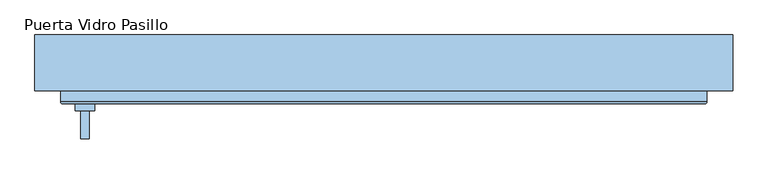
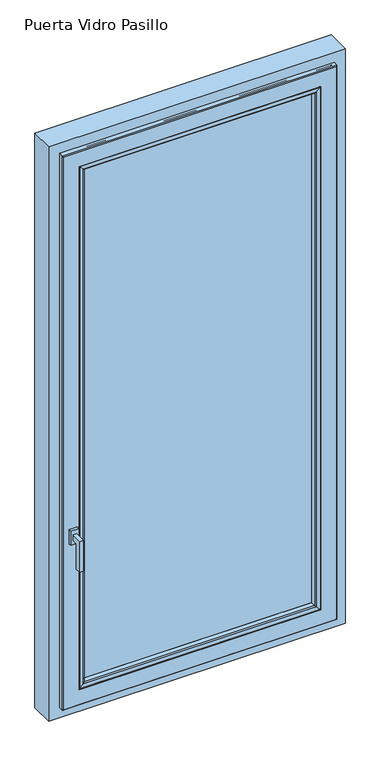
"""IFC4 building model written with IfcOpenShell, lengths in millimetres: window geometry, 2019_ES_Ventana_Replus_re80pvc301_10100_1-Hoja : Puerta Vidro Pasillo."""

from ifc_helpers import new_model, si_unit, frame, origin, place, context, project, spatial, polyline, ellipse_curve, outline, extrude, source, transform, mapped, element, save
from ifc_brep_helpers import plane_surface, cylinder_surface, advanced_brep


def puerta_vidro_pasillo_571ac3f6(model_context):
    return source(origin(), model_context, "Body", "SolidModel", [
        extrude(outline(polyline([(-78.4999991, 1470.0), (-78.4999991, 1450.0), (-98.4999991, 1450.0), (-98.4999991, 1360.0), (-118.4999991, 1360.0), (-118.4999991, 1470.0), (-78.4999991, 1470.0)])), frame((-434.1999993, 0.0, 0.0), z_axis=(1.0, 0.0, 0.0), x_axis=(0.0, 1.0, 0.0)), (0.0, 0.0, 1.0), 12.0),
        extrude(outline(polyline([(-413.9687607, -78.4999991), (-442.4312378, -78.4999991), (-442.4312378, -68.4999991), (-413.9687607, -68.4999991), (-413.9687607, -78.4999991)])), frame((0.0, 0.0, 1435.217127), z_axis=(0.0, 0.0, 1.0), x_axis=(1.0, 0.0, 0.0)), (0.0, 0.0, 1.0), 49.565746),
        extrude(outline(polyline([(2757.2, 397.1999993), (2757.2, -397.1999993), (909.8, -397.1999993), (909.8, 397.1999993), (2757.2, 397.1999993)]), holes=[polyline([(917.8, 389.1999993), (917.8, -389.1999993), (2749.2, -389.1999993), (2749.2, 389.1999993), (917.8, 389.1999993)])]), frame((0.0, -26.9999999, 0.0), z_axis=(0.0, 1.0, 0.0), x_axis=(0.0, 0.0, 1.0)), (0.0, 0.0, 1.0), 16.0),
        extrude(outline(polyline([(2757.1868066, 397.1868058), (2757.1868066, -397.1868058), (909.8131934, -397.1868058), (909.8131934, 397.1868058), (2757.1868066, 397.1868058)]), holes=[polyline([(917.8, 389.1999993), (917.8, -389.1999993), (2749.2, -389.1999993), (2749.2, 389.1999993), (917.8, 389.1999993)])]), frame((0.0, -47.0000001, 0.0), z_axis=(0.0, 1.0, 0.0), x_axis=(0.0, 0.0, 1.0)), (0.0, 0.0, 1.0), 16.0),
        extrude(outline(polyline([(397.1999993, -6.9999997), (397.1999993, -10.9999999), (-397.1999993, -10.9999999), (-397.1999993, -6.9999997), (397.1999993, -6.9999997)])), frame((0.0, 0.0, 903.7946451), z_axis=(0.0, 0.0, 1.0), x_axis=(1.0, 0.0, 0.0)), (0.0, 0.0, 1.0), 1859.4053549),
        extrude(outline(polyline([(397.1999993, -26.9999999), (397.1999993, -31.0000001), (-397.1999993, -31.0000001), (-397.1999993, -26.9999999), (397.1999993, -26.9999999)])), frame((0.0, 0.0, 903.7946451), z_axis=(0.0, 0.0, 1.0), x_axis=(1.0, 0.0, 0.0)), (0.0, 0.0, 1.0), 1859.4053549),
        extrude(outline(polyline([(397.1999993, -47.0000001), (397.1999993, -51.0000003), (-397.1999993, -51.0000003), (-397.1999993, -47.0000001), (397.1999993, -47.0000001)])), frame((0.0, 0.0, 903.7946451), z_axis=(0.0, 0.0, 1.0), x_axis=(1.0, 0.0, 0.0)), (0.0, 0.0, 1.0), 1859.4053549),
        advanced_brep(
        [(387.2913171, 9.2764571, 2747.2913178), (390.1890946, 11.5, 2750.1890953), (390.1890946, 11.5, 919.8109047), (387.2913171, 9.2764571, 922.7086822), (430.1999993, 11.5, 879.8), (-430.1999993, 11.5, 879.8), (-430.1999993, 11.5, 2790.2), (430.1999993, 11.5, 2790.2), (-390.1890946, 11.5, 2750.1890953), (-390.1890946, 11.5, 919.8109047), (-387.2913171, 9.2764571, 922.7086822), (384.1757968, -2.3508228, 2744.1757976), (384.1757968, -2.3508228, 925.8242024), (-384.1757968, -2.3508228, 925.8242024), (384.6739305, -3.0000033, 2744.6739313), (384.6739305, -3.0000033, 925.3260687), (-384.6739305, -3.0000033, 925.3260687), (391.1999993, -3.0000033, 2751.2), (-391.1999993, -3.0000033, 2751.2), (-391.1999993, -3.0000033, 918.8), (391.1999993, -3.0000033, 918.8), (-384.6739305, -3.0000033, 2744.6739313), (391.1999993, -6.9999997, 2751.2), (391.1999993, -6.9999997, 918.8), (-391.1999993, -6.9999997, 918.8), (411.8162192, -6.9999997, 2771.8162199), (-411.8162192, -6.9999997, 2771.8162199), (-411.8162192, -6.9999997, 898.1837801), (411.8162192, -6.9999997, 898.1837801), (-391.1999993, -6.9999997, 2751.2), (409.1999993, -25.6153717, 2769.2), (409.1999993, -25.6153717, 900.8), (-409.1999993, -25.6153717, 900.8), (409.1999993, -56.4999995, 2769.2), (409.1999993, -56.4999995, 900.8), (-409.1999993, -56.4999995, 900.8), (-409.1999993, -56.4999995, 2769.2), (397.1999993, -56.4999995, 2757.2), (-397.1999993, -56.4999995, 2757.2), (-397.1999993, -56.4999995, 912.8), (397.1999993, -56.4999995, 912.8), (397.1999993, -51.0000003, 2757.2), (397.1999993, -51.0000003, 912.8), (-397.1999993, -51.0000003, 912.8), (-397.1999993, -51.0000003, 2757.2), (386.007687, -51.0000003, 2746.0076877), (-386.007687, -51.0000003, 2746.0076877), (-386.007687, -51.0000003, 923.9923123), (386.007687, -51.0000003, 923.9923123), (385.4940999, -51.6693201, 2745.4941006), (385.4940999, -51.6693201, 924.5058994), (-385.4940999, -51.6693201, 924.5058994), (388.8993918, -64.3780426, 2748.8993925), (388.8993918, -64.3780426, 921.1006075), (-388.8993918, -64.3780426, 921.1006075), (392.6234971, -67.3403297, 2752.6234978), (392.6234971, -67.3403297, 917.3765022), (-392.6234971, -67.3403297, 917.3765022), (405.6488427, -67.7951848, 2765.6488434), (405.6488427, -67.7951848, 904.3511566), (-405.6488427, -67.7951848, 904.3511566), (406.1999993, -67.2629391, 2766.2), (406.1999993, -67.2629391, 903.8), (-406.1999993, -67.2629391, 903.8), (407.4370593, -68.4999991, 2767.43706), (407.4370593, -68.4999991, 902.56294), (-407.4370593, -68.4999991, 902.56294), (460.1999993, -68.4999991, 2820.2), (-460.1999993, -68.4999991, 2820.2), (-460.1999993, -68.4999991, 849.8), (460.1999993, -68.4999991, 849.8), (-407.4370593, -68.4999991, 2767.43706), (463.1999993, -65.4999991, 2823.2), (463.1999993, -65.4999991, 846.8), (-463.1999993, -65.4999991, 846.8), (463.1999993, -50.0, 2823.2), (463.1999993, -50.0, 846.8), (-463.1999993, -50.0, 846.8), (-463.1999993, -50.0, 2823.2), (443.1999993, -50.0, 2803.2), (-443.1999993, -50.0, 2803.2), (-443.1999993, -50.0, 866.8), (443.1999993, -50.0, 866.8), (443.1999993, -11.9999991, 866.8), (443.1999993, -11.9999991, 2803.2), (-443.1999993, -11.9999991, 866.8), (-443.1999993, -11.9999991, 2803.2), (430.1999993, -11.9999991, 2790.2), (-430.1999993, -11.9999991, 2790.2), (-430.1999993, -11.9999991, 879.8), (430.1999993, -11.9999991, 879.8), (-387.2913171, 9.2764571, 2747.2913178), (-384.1757968, -2.3508228, 2744.1757976), (-409.1999993, -25.6153717, 2769.2), (-385.4940999, -51.6693201, 2745.4941006), (-388.8993918, -64.3780426, 2748.8993925), (-392.6234971, -67.3403297, 2752.6234978), (-405.6488427, -67.7951848, 2765.6488434), (-406.1999993, -67.2629391, 2766.2), (-463.1999993, -65.4999991, 2823.2)],
        [
            (0, 1, ellipse_curve(frame((390.1890946, 8.5, 2750.1890953), z_axis=(0.7071067811865475, 0.0, -0.7071067811865475), x_axis=(0.7071067811865474, 0.0, 0.7071067811865476)), 4.2426407, 3.0)),
            (1, 2),
            (2, 3, ellipse_curve(frame((390.1890946, 8.5, 919.8109047), z_axis=(0.7071067811865475, 0.0, 0.7071067811865475), x_axis=(-0.7071067811865474, 0.0, 0.7071067811865476)), 4.2426407, 3.0)),
            (3, 0),
            (4, 5),
            (5, 6),
            (6, 7),
            (7, 4),
            (1, 8),
            (8, 9),
            (9, 2),
            (9, 10, ellipse_curve(frame((-390.1890946, 8.5, 919.8109047), z_axis=(0.7071067811865475, 0.0, -0.7071067811865475), x_axis=(0.7071067811865476, 0.0, 0.7071067811865474)), 4.2426407, 3.0)),
            (10, 3),
            (11, 0),
            (3, 12),
            (12, 11),
            (10, 13),
            (13, 12),
            (14, 11, ellipse_curve(frame((384.6739305, -2.4842973, 2744.6739313), z_axis=(0.7071067811865475, 0.0, -0.7071067811865475), x_axis=(0.7071067811865474, 0.0, 0.7071067811865476)), 0.7293184, 0.515706)),
            (12, 15, ellipse_curve(frame((384.6739305, -2.4842973, 925.3260687), z_axis=(0.7071067811865475, 0.0, 0.7071067811865475), x_axis=(-0.7071067811865474, 0.0, 0.7071067811865476)), 0.7293184, 0.515706)),
            (15, 14),
            (13, 16, ellipse_curve(frame((-384.6739305, -2.4842973, 925.3260687), z_axis=(0.7071067811865475, 0.0, -0.7071067811865475), x_axis=(0.7071067811865476, 0.0, 0.7071067811865474)), 0.7293184, 0.515706)),
            (16, 15),
            (17, 18),
            (18, 19),
            (19, 20),
            (20, 17),
            (16, 21),
            (21, 14),
            (22, 17),
            (20, 23),
            (23, 22),
            (19, 24),
            (24, 23),
            (25, 26),
            (26, 27),
            (27, 28),
            (28, 25),
            (24, 29),
            (29, 22),
            (30, 25),
            (28, 31),
            (31, 30),
            (27, 32),
            (32, 31),
            (33, 30),
            (31, 34),
            (34, 33),
            (32, 35),
            (35, 34),
            (35, 36),
            (36, 33),
            (37, 38),
            (38, 39),
            (39, 40),
            (40, 37),
            (41, 37),
            (40, 42),
            (42, 41),
            (39, 43),
            (43, 42),
            (43, 44),
            (44, 41),
            (45, 46),
            (46, 47),
            (47, 48),
            (48, 45),
            (49, 45, ellipse_curve(frame((386.007687, -51.5317048, 2746.0076877), z_axis=(0.7071067811865475, 0.0, -0.7071067811865475), x_axis=(0.7071067811865474, 0.0, 0.7071067811865476)), 0.7519437, 0.5317045)),
            (48, 50, ellipse_curve(frame((386.007687, -51.5317048, 923.9923123), z_axis=(0.7071067811865475, 0.0, 0.7071067811865475), x_axis=(-0.7071067811865474, 0.0, 0.7071067811865476)), 0.7519437, 0.5317045)),
            (50, 49),
            (47, 51, ellipse_curve(frame((-386.007687, -51.5317048, 923.9923123), z_axis=(0.7071067811865475, 0.0, -0.7071067811865475), x_axis=(0.7071067811865476, 0.0, 0.7071067811865474)), 0.7519437, 0.5317045)),
            (51, 50),
            (52, 49),
            (50, 53),
            (53, 52),
            (51, 54),
            (54, 53),
            (55, 52, ellipse_curve(frame((392.7630951, -63.3427664, 2752.7630958), z_axis=(0.7071067811865475, 0.0, -0.7071067811865475), x_axis=(0.7071067811865474, 0.0, 0.7071067811865476)), 5.6568542, 4.0)),
            (53, 56, ellipse_curve(frame((392.7630951, -63.3427664, 917.2369042), z_axis=(0.7071067811865475, 0.0, 0.7071067811865475), x_axis=(-0.7071067811865474, 0.0, 0.7071067811865476)), 5.6568542, 4.0)),
            (56, 55),
            (54, 57, ellipse_curve(frame((-392.7630951, -63.3427664, 917.2369042), z_axis=(0.7071067811865475, 0.0, -0.7071067811865475), x_axis=(0.7071067811865476, 0.0, 0.7071067811865474)), 5.6568542, 4.0)),
            (57, 56),
            (58, 55),
            (56, 59),
            (59, 58),
            (57, 60),
            (60, 59),
            (61, 58, ellipse_curve(frame((405.6674291, -67.2629391, 2765.6674299), z_axis=(0.7071067811865475, 0.0, -0.7071067811865475), x_axis=(0.7071067811865474, 0.0, 0.7071067811865476)), 0.7531679, 0.5325701)),
            (59, 62, ellipse_curve(frame((405.6674291, -67.2629391, 904.3325701), z_axis=(0.7071067811865475, 0.0, 0.7071067811865475), x_axis=(-0.7071067811865474, 0.0, 0.7071067811865476)), 0.7531679, 0.5325701)),
            (62, 61),
            (60, 63, ellipse_curve(frame((-405.6674291, -67.2629391, 904.3325701), z_axis=(0.7071067811865475, 0.0, -0.7071067811865475), x_axis=(0.7071067811865476, 0.0, 0.7071067811865474)), 0.7531679, 0.5325701)),
            (63, 62),
            (64, 61, ellipse_curve(frame((407.4370593, -67.2629391, 2767.43706), z_axis=(0.7071067811865475, 0.0, -0.7071067811865475), x_axis=(0.7071067811865474, 0.0, 0.7071067811865476)), 1.7494671, 1.23706)),
            (62, 65, ellipse_curve(frame((407.4370593, -67.2629391, 902.56294), z_axis=(0.7071067811865475, 0.0, 0.7071067811865475), x_axis=(-0.7071067811865474, 0.0, 0.7071067811865476)), 1.7494671, 1.23706)),
            (65, 64),
            (63, 66, ellipse_curve(frame((-407.4370593, -67.2629391, 902.56294), z_axis=(0.7071067811865475, 0.0, -0.7071067811865475), x_axis=(0.7071067811865476, 0.0, 0.7071067811865474)), 1.7494671, 1.23706)),
            (66, 65),
            (67, 68),
            (68, 69),
            (69, 70),
            (70, 67),
            (66, 71),
            (71, 64),
            (72, 67, ellipse_curve(frame((460.1999993, -65.4999991, 2820.2), z_axis=(0.7071067811865475, 0.0, -0.7071067811865475), x_axis=(0.7071067811865474, 0.0, 0.7071067811865476)), 4.2426407, 3.0)),
            (70, 73, ellipse_curve(frame((460.1999993, -65.4999991, 849.8), z_axis=(0.7071067811865475, 0.0, 0.7071067811865475), x_axis=(-0.7071067811865474, 0.0, 0.7071067811865476)), 4.2426407, 3.0)),
            (73, 72),
            (69, 74, ellipse_curve(frame((-460.1999993, -65.4999991, 849.8), z_axis=(0.7071067811865475, 0.0, -0.7071067811865475), x_axis=(0.7071067811865476, 0.0, 0.7071067811865474)), 4.2426407, 3.0)),
            (74, 73),
            (75, 72),
            (73, 76),
            (76, 75),
            (74, 77),
            (77, 76),
            (77, 78),
            (78, 75),
            (79, 80),
            (80, 81),
            (81, 82),
            (82, 79),
            (82, 83),
            (83, 84),
            (84, 79),
            (81, 85),
            (85, 83),
            (85, 86),
            (86, 84),
            (87, 88),
            (88, 89),
            (89, 90),
            (90, 87),
            (90, 4),
            (7, 87),
            (89, 5),
            (8, 91, ellipse_curve(frame((-390.1890946, 8.5, 2750.1890953), z_axis=(-0.7071067811865475, 0.0, -0.7071067811865475), x_axis=(0.7071067811865474, 0.0, -0.7071067811865476)), 4.2426407, 3.0)),
            (91, 10),
            (91, 92),
            (92, 13),
            (92, 21, ellipse_curve(frame((-384.6739305, -2.4842973, 2744.6739313), z_axis=(-0.7071067811865475, 0.0, -0.7071067811865475), x_axis=(0.7071067811865474, 0.0, -0.7071067811865476)), 0.7293184, 0.515706)),
            (18, 29),
            (26, 93),
            (93, 32),
            (93, 36),
            (38, 44),
            (46, 94, ellipse_curve(frame((-386.007687, -51.5317048, 2746.0076877), z_axis=(-0.7071067811865475, 0.0, -0.7071067811865475), x_axis=(0.7071067811865474, 0.0, -0.7071067811865476)), 0.7519437, 0.5317045)),
            (94, 51),
            (94, 95),
            (95, 54),
            (95, 96, ellipse_curve(frame((-392.7630951, -63.3427664, 2752.7630958), z_axis=(-0.7071067811865475, 0.0, -0.7071067811865475), x_axis=(0.7071067811865474, 0.0, -0.7071067811865476)), 5.6568542, 4.0)),
            (96, 57),
            (96, 97),
            (97, 60),
            (97, 98, ellipse_curve(frame((-405.6674291, -67.2629391, 2765.6674299), z_axis=(-0.7071067811865475, 0.0, -0.7071067811865475), x_axis=(0.7071067811865474, 0.0, -0.7071067811865476)), 0.7531679, 0.5325701)),
            (98, 63),
            (98, 71, ellipse_curve(frame((-407.4370593, -67.2629391, 2767.43706), z_axis=(-0.7071067811865475, 0.0, -0.7071067811865475), x_axis=(0.7071067811865474, 0.0, -0.7071067811865476)), 1.7494671, 1.23706)),
            (68, 99, ellipse_curve(frame((-460.1999993, -65.4999991, 2820.2), z_axis=(-0.7071067811865475, 0.0, -0.7071067811865475), x_axis=(0.7071067811865474, 0.0, -0.7071067811865476)), 4.2426407, 3.0)),
            (99, 74),
            (99, 78),
            (80, 86),
            (88, 6),
            (0, 91),
            (11, 92),
            (30, 93),
            (49, 94),
            (52, 95),
            (55, 96),
            (58, 97),
            (61, 98),
            (72, 99),
        ],
        [
            cylinder_surface(frame((390.1890946, 8.5, 2823.2), z_axis=(0.0, 0.0, 1.0), x_axis=(-1.0, 0.0, 0.0)), 3.0),
            plane_surface(frame((-430.1999993, 11.5, 2790.2), z_axis=(0.0, 1.0, 0.0), x_axis=(1.0, 0.0, 0.0))),
            cylinder_surface(frame((463.1999993, 8.5, 919.8109047), z_axis=(1.0, 0.0, 0.0), x_axis=(0.0, 0.0, 1.0)), 3.0),
            plane_surface(frame((387.2913171, 9.2764571, 2747.2913178), z_axis=(-0.9659258263570549, 0.2588190448487916, 0.0), x_axis=(0.0, 0.0, -1.0))),
            plane_surface(frame((387.2913171, 9.2764571, 922.7086822), z_axis=(0.0, 0.2588190448487885, 0.9659258263570558), x_axis=(-1.0, 0.0, 0.0))),
            cylinder_surface(frame((384.6739305, -2.4842973, 2823.2), z_axis=(0.0, 0.0, 1.0), x_axis=(-1.0, 0.0, 0.0)), 0.515706),
            cylinder_surface(frame((463.1999993, -2.4842973, 925.3260687), z_axis=(1.0, 0.0, 0.0), x_axis=(0.0, 0.0, 1.0)), 0.515706),
            plane_surface(frame((-384.6739305, -3.0000033, 2744.6739313), z_axis=(0.0, -1.0, 0.0), x_axis=(1.0, 0.0, 0.0))),
            plane_surface(frame((391.1999993, -3.0000033, 2751.2), z_axis=(-1.0, 0.0, 0.0), x_axis=(0.0, 0.0, -1.0))),
            plane_surface(frame((391.1999993, -3.0000033, 918.8), z_axis=(0.0, 0.0, 1.0), x_axis=(-1.0, 0.0, 0.0))),
            plane_surface(frame((-391.1999993, -6.9999997, 2751.2), z_axis=(0.0, -1.0, 0.0), x_axis=(1.0, 0.0, 0.0))),
            plane_surface(frame((411.8162192, -6.9999997, 2771.8162199), z_axis=(-0.9902680687415736, 0.13917310096004265, 0.0), x_axis=(0.0, 0.0, -1.0))),
            plane_surface(frame((411.8162192, -6.9999997, 898.1837801), z_axis=(0.0, 0.13917310096003946, 0.990268068741574), x_axis=(-1.0, 0.0, 0.0))),
            plane_surface(frame((409.1999993, -25.6153717, 2769.2), z_axis=(-1.0, 0.0, 0.0), x_axis=(0.0, 0.0, -1.0))),
            plane_surface(frame((409.1999993, -25.6153717, 900.8), z_axis=(0.0, 0.0, 1.0), x_axis=(-1.0, 0.0, 0.0))),
            plane_surface(frame((-409.1999993, -56.4999995, 2769.2), z_axis=(0.0, 1.0, 0.0), x_axis=(1.0, 0.0, 0.0))),
            plane_surface(frame((397.1999993, -56.4999995, 2757.2), z_axis=(1.0, 0.0, 0.0), x_axis=(0.0, 0.0, -1.0))),
            plane_surface(frame((397.1999993, -56.4999995, 912.8), z_axis=(0.0, 0.0, -1.0), x_axis=(-1.0, 0.0, 0.0))),
            plane_surface(frame((-397.1999993, -51.0000003, 2757.2), z_axis=(0.0, 1.0, 0.0), x_axis=(1.0, 0.0, 0.0))),
            cylinder_surface(frame((386.007687, -51.5317048, 2823.2), z_axis=(0.0, 0.0, 1.0), x_axis=(-1.0, 0.0, 0.0)), 0.5317045),
            cylinder_surface(frame((463.1999993, -51.5317048, 923.9923123), z_axis=(1.0, 0.0, 0.0), x_axis=(0.0, 0.0, 1.0)), 0.5317045),
            plane_surface(frame((385.4940999, -51.6693201, 2745.4941006), z_axis=(-0.9659258262890666, -0.2588190451025272, 0.0), x_axis=(0.0, 0.0, -1.0))),
            plane_surface(frame((385.4940999, -51.6693201, 924.5058994), z_axis=(0.0, -0.2588190451025303, 0.9659258262890658), x_axis=(-1.0, 0.0, 0.0))),
            cylinder_surface(frame((392.7630951, -63.3427664, 2823.2), z_axis=(0.0, 0.0, 1.0), x_axis=(-1.0, 0.0, 0.0)), 4.0),
            cylinder_surface(frame((463.1999993, -63.3427664, 917.2369042), z_axis=(1.0, 0.0, 0.0), x_axis=(0.0, 0.0, 1.0)), 4.0),
            plane_surface(frame((392.6234971, -67.3403297, 2752.6234978), z_axis=(-0.034899496702507804, -0.9993908270190955, 0.0), x_axis=(0.0, 0.0, -1.0))),
            plane_surface(frame((392.6234971, -67.3403297, 917.3765022), z_axis=(0.0, -0.9993908270190957, 0.03489949670250457), x_axis=(-1.0, 0.0, 0.0))),
            cylinder_surface(frame((405.6674291, -67.2629391, 2823.2), z_axis=(0.0, 0.0, 1.0), x_axis=(-1.0, 0.0, 0.0)), 0.5325701),
            cylinder_surface(frame((463.1999993, -67.2629391, 904.3325701), z_axis=(1.0, 0.0, 0.0), x_axis=(0.0, 0.0, 1.0)), 0.5325701),
            cylinder_surface(frame((407.4370593, -67.2629391, 2823.2), z_axis=(0.0, 0.0, 1.0), x_axis=(-1.0, 0.0, 0.0)), 1.23706),
            cylinder_surface(frame((463.1999993, -67.2629391, 902.56294), z_axis=(1.0, 0.0, 0.0), x_axis=(0.0, 0.0, 1.0)), 1.23706),
            plane_surface(frame((-407.4370593, -68.4999991, 2767.43706), z_axis=(0.0, -1.0, 0.0), x_axis=(1.0, 0.0, 0.0))),
            cylinder_surface(frame((460.1999993, -65.4999991, 2823.2), z_axis=(0.0, 0.0, 1.0), x_axis=(-1.0, 0.0, 0.0)), 3.0),
            cylinder_surface(frame((463.1999993, -65.4999991, 849.8), z_axis=(1.0, 0.0, 0.0), x_axis=(0.0, 0.0, 1.0)), 3.0),
            plane_surface(frame((463.1999993, -65.4999991, 2823.2), z_axis=(1.0, 0.0, 0.0), x_axis=(0.0, 0.0, -1.0))),
            plane_surface(frame((463.1999993, -65.4999991, 846.8), z_axis=(0.0, 0.0, -1.0), x_axis=(-1.0, 0.0, 0.0))),
            plane_surface(frame((-459.2000019, -50.0, 2819.2000027), z_axis=(0.0, 1.0, 0.0), x_axis=(1.0, 0.0, 0.0))),
            plane_surface(frame((443.1999993, -45.0999991, 2803.2), z_axis=(1.0, 0.0, 0.0), x_axis=(0.0, 0.0, -1.0))),
            plane_surface(frame((443.1999993, -45.0999991, 866.8), z_axis=(0.0, 0.0, -1.0), x_axis=(-1.0, 0.0, 0.0))),
            plane_surface(frame((-435.7000002, -11.9999991, 2795.7000009), z_axis=(0.0, 1.0, 0.0), x_axis=(1.0, 0.0, 0.0))),
            plane_surface(frame((430.1999993, -1.4999991, 2790.2), z_axis=(1.0, 0.0, 0.0), x_axis=(0.0, 0.0, -1.0))),
            plane_surface(frame((430.1999993, -1.4999991, 879.8), z_axis=(0.0, 0.0, -1.0), x_axis=(-1.0, 0.0, 0.0))),
            cylinder_surface(frame((-390.1890946, 8.5, 846.8), z_axis=(0.0, 0.0, -1.0), x_axis=(1.0, 0.0, 0.0)), 3.0),
            plane_surface(frame((-387.2913171, 9.2764571, 922.7086822), z_axis=(0.9659258263570565, 0.2588190448487853, 0.0), x_axis=(0.0, 0.0, 1.0))),
            cylinder_surface(frame((-384.6739305, -2.4842973, 846.8), z_axis=(0.0, 0.0, -1.0), x_axis=(1.0, 0.0, 0.0)), 0.515706),
            plane_surface(frame((-391.1999993, -3.0000033, 918.8), z_axis=(1.0, 0.0, 0.0), x_axis=(0.0, 0.0, 1.0))),
            plane_surface(frame((-411.8162192, -6.9999997, 898.1837801), z_axis=(0.9902680687415745, 0.13917310096003627, 0.0), x_axis=(0.0, 0.0, 1.0))),
            plane_surface(frame((-409.1999993, -25.6153717, 900.8), z_axis=(1.0, 0.0, 0.0), x_axis=(0.0, 0.0, 1.0))),
            plane_surface(frame((-397.1999993, -56.4999995, 912.8), z_axis=(-1.0, 0.0, 0.0), x_axis=(0.0, 0.0, 1.0))),
            cylinder_surface(frame((-386.007687, -51.5317048, 846.8), z_axis=(0.0, 0.0, -1.0), x_axis=(1.0, 0.0, 0.0)), 0.5317045),
            plane_surface(frame((-385.4940999, -51.6693201, 924.5058994), z_axis=(0.9659258262890649, -0.2588190451025334, 0.0), x_axis=(0.0, 0.0, 1.0))),
            cylinder_surface(frame((-392.7630951, -63.3427664, 846.8), z_axis=(0.0, 0.0, -1.0), x_axis=(1.0, 0.0, 0.0)), 4.0),
            plane_surface(frame((-392.6234971, -67.3403297, 917.3765022), z_axis=(0.03489949670250134, -0.9993908270190958, 0.0), x_axis=(0.0, 0.0, 1.0))),
            cylinder_surface(frame((-405.6674291, -67.2629391, 846.8), z_axis=(0.0, 0.0, -1.0), x_axis=(1.0, 0.0, 0.0)), 0.5325701),
            cylinder_surface(frame((-407.4370593, -67.2629391, 846.8), z_axis=(0.0, 0.0, -1.0), x_axis=(1.0, 0.0, 0.0)), 1.23706),
            cylinder_surface(frame((-460.1999993, -65.4999991, 846.8), z_axis=(0.0, 0.0, -1.0), x_axis=(1.0, 0.0, 0.0)), 3.0),
            plane_surface(frame((-463.1999993, -65.4999991, 846.8), z_axis=(-1.0, 0.0, 0.0), x_axis=(0.0, 0.0, 1.0))),
            plane_surface(frame((-443.1999993, -45.0999991, 866.8), z_axis=(-1.0, 0.0, 0.0), x_axis=(0.0, 0.0, 1.0))),
            plane_surface(frame((-430.1999993, -1.4999991, 879.8), z_axis=(-1.0, 0.0, 0.0), x_axis=(0.0, 0.0, 1.0))),
            cylinder_surface(frame((-463.1999993, 8.5, 2750.1890953), z_axis=(-1.0, 0.0, 0.0), x_axis=(0.0, 0.0, -1.0)), 3.0),
            plane_surface(frame((-387.2913171, 9.2764571, 2747.2913178), z_axis=(0.0, 0.2588190448487885, -0.9659258263570557), x_axis=(1.0, 0.0, 0.0))),
            cylinder_surface(frame((-463.1999993, -2.4842973, 2744.6739313), z_axis=(-1.0, 0.0, 0.0), x_axis=(0.0, 0.0, -1.0)), 0.515706),
            plane_surface(frame((-391.1999993, -3.0000033, 2751.2), z_axis=(0.0, 0.0, -1.0), x_axis=(1.0, 0.0, 0.0))),
            plane_surface(frame((-411.8162192, -6.9999997, 2771.8162199), z_axis=(0.0, 0.13917310096003946, -0.990268068741574), x_axis=(1.0, 0.0, 0.0))),
            plane_surface(frame((-409.1999993, -25.6153717, 2769.2), z_axis=(0.0, 0.0, -1.0), x_axis=(1.0, 0.0, 0.0))),
            plane_surface(frame((-397.1999993, -56.4999995, 2757.2), z_axis=(0.0, 0.0, 1.0), x_axis=(1.0, 0.0, 0.0))),
            cylinder_surface(frame((-463.1999993, -51.5317048, 2746.0076877), z_axis=(-1.0, 0.0, 0.0), x_axis=(0.0, 0.0, -1.0)), 0.5317045),
            plane_surface(frame((-385.4940999, -51.6693201, 2745.4941006), z_axis=(0.0, -0.2588190451025303, -0.9659258262890658), x_axis=(1.0, 0.0, 0.0))),
            cylinder_surface(frame((-463.1999993, -63.3427664, 2752.7630958), z_axis=(-1.0, 0.0, 0.0), x_axis=(0.0, 0.0, -1.0)), 4.0),
            plane_surface(frame((-392.6234971, -67.3403297, 2752.6234978), z_axis=(0.0, -0.9993908270190957, -0.03489949670250457), x_axis=(1.0, 0.0, 0.0))),
            cylinder_surface(frame((-463.1999993, -67.2629391, 2765.6674299), z_axis=(-1.0, 0.0, 0.0), x_axis=(0.0, 0.0, -1.0)), 0.5325701),
            cylinder_surface(frame((-463.1999993, -67.2629391, 2767.43706), z_axis=(-1.0, 0.0, 0.0), x_axis=(0.0, 0.0, -1.0)), 1.23706),
            cylinder_surface(frame((-463.1999993, -65.4999991, 2820.2), z_axis=(-1.0, 0.0, 0.0), x_axis=(0.0, 0.0, -1.0)), 3.0),
            plane_surface(frame((-463.1999993, -65.4999991, 2823.2), z_axis=(0.0, 0.0, 1.0), x_axis=(1.0, 0.0, 0.0))),
            plane_surface(frame((-443.1999993, -45.0999991, 2803.2), z_axis=(0.0, 0.0, 1.0), x_axis=(1.0, 0.0, 0.0))),
            plane_surface(frame((-430.1999993, -1.4999991, 2790.2), z_axis=(0.0, 0.0, 1.0), x_axis=(1.0, 0.0, 0.0))),
        ],
        [
            (0, [[1, 2, 3, 4]]),
            (1, [[5, 6, 7, 8], [9, 10, 11, -2]]),
            (2, [[-3, -11, 12, 13]]),
            (3, [[14, -4, 15, 16]]),
            (4, [[-15, -13, 17, 18]]),
            (5, [[19, -16, 20, 21]]),
            (6, [[-20, -18, 22, 23]]),
            (7, [[24, 25, 26, 27], [-23, 28, 29, -21]]),
            (8, [[30, -27, 31, 32]]),
            (9, [[-31, -26, 33, 34]]),
            (10, [[35, 36, 37, 38], [-34, 39, 40, -32]]),
            (11, [[41, -38, 42, 43]]),
            (12, [[-42, -37, 44, 45]]),
            (13, [[46, -43, 47, 48]]),
            (14, [[-47, -45, 49, 50]]),
            (15, [[-50, 51, 52, -48], [53, 54, 55, 56]]),
            (16, [[57, -56, 58, 59]]),
            (17, [[-58, -55, 60, 61]]),
            (18, [[-61, 62, 63, -59], [64, 65, 66, 67]]),
            (19, [[68, -67, 69, 70]]),
            (20, [[-69, -66, 71, 72]]),
            (21, [[73, -70, 74, 75]]),
            (22, [[-74, -72, 76, 77]]),
            (23, [[78, -75, 79, 80]]),
            (24, [[-79, -77, 81, 82]]),
            (25, [[83, -80, 84, 85]]),
            (26, [[-84, -82, 86, 87]]),
            (27, [[88, -85, 89, 90]]),
            (28, [[-89, -87, 91, 92]]),
            (29, [[93, -90, 94, 95]]),
            (30, [[-94, -92, 96, 97]]),
            (31, [[98, 99, 100, 101], [-97, 102, 103, -95]]),
            (32, [[104, -101, 105, 106]]),
            (33, [[-105, -100, 107, 108]]),
            (34, [[109, -106, 110, 111]]),
            (35, [[-110, -108, 112, 113]]),
            (36, [[-113, 114, 115, -111], [116, 117, 118, 119]]),
            (37, [[-119, 120, 121, 122]]),
            (38, [[-120, -118, 123, 124]]),
            (39, [[-124, 125, 126, -121], [127, 128, 129, 130]]),
            (40, [[-130, 131, -8, 132]]),
            (41, [[-131, -129, 133, -5]]),
            (42, [[-12, -10, 134, 135]]),
            (43, [[-17, -135, 136, 137]]),
            (44, [[-22, -137, 138, -28]]),
            (45, [[-33, -25, 139, -39]]),
            (46, [[-44, -36, 140, 141]]),
            (47, [[-49, -141, 142, -51]]),
            (48, [[-60, -54, 143, -62]]),
            (49, [[-71, -65, 144, 145]]),
            (50, [[-76, -145, 146, 147]]),
            (51, [[-81, -147, 148, 149]]),
            (52, [[-86, -149, 150, 151]]),
            (53, [[-91, -151, 152, 153]]),
            (54, [[-96, -153, 154, -102]]),
            (55, [[-107, -99, 155, 156]]),
            (56, [[-112, -156, 157, -114]]),
            (57, [[-123, -117, 158, -125]]),
            (58, [[-133, -128, 159, -6]]),
            (59, [[-134, -9, -1, 160]]),
            (60, [[-136, -160, -14, 161]]),
            (61, [[-138, -161, -19, -29]]),
            (62, [[-139, -24, -30, -40]]),
            (63, [[-140, -35, -41, 162]]),
            (64, [[-142, -162, -46, -52]]),
            (65, [[-143, -53, -57, -63]]),
            (66, [[-144, -64, -68, 163]]),
            (67, [[-146, -163, -73, 164]]),
            (68, [[-148, -164, -78, 165]]),
            (69, [[-150, -165, -83, 166]]),
            (70, [[-152, -166, -88, 167]]),
            (71, [[-154, -167, -93, -103]]),
            (72, [[-155, -98, -104, 168]]),
            (73, [[-157, -168, -109, -115]]),
            (74, [[-158, -116, -122, -126]]),
            (75, [[-159, -127, -132, -7]]),
        ],
    ),
        advanced_brep(
        [(423.2673545, 12.758819, 2783.2673545), (427.2913185, 27.7764571, 2787.2913185), (427.2913185, 27.7764571, 882.7086815), (423.2673545, 12.758819, 886.7326455), (430.189096, 30.0, 2790.189096), (430.189096, 30.0, 879.810904), (-427.2913185, 27.7764571, 882.7086815), (-423.2673545, 12.758819, 886.7326455), (424.2332803, 11.5, 2784.2332803), (424.2332803, 11.5, 885.7667197), (500.0, 30.0, 2860.0), (500.0, -50.0, 2860.0), (500.0, -50.0, 810.0), (500.0, 30.0, 810.0), (-500.0, -50.0, 2860.0), (-500.0, -50.0, 810.0), (456.1999993, -50.0, 853.8000007), (-456.1999993, -50.0, 853.8000007), (-456.1999993, -50.0, 2816.1999993), (456.1999993, -50.0, 2816.1999993), (-500.0, 30.0, 810.0), (-500.0, 30.0, 2860.0), (-430.189096, 30.0, 2790.189096), (-430.189096, 30.0, 879.810904), (436.1891471, -8.0, 2796.1891471), (436.1891471, 11.5, 2796.1891471), (436.1891471, 11.5, 873.8108529), (436.1891471, -8.0, 873.8108529), (-436.1891471, 11.5, 2796.1891471), (-436.1891471, 11.5, 873.8108529), (-424.2332803, 11.5, 885.7667197), (-424.2332803, 11.5, 2784.2332803), (-436.1891471, -8.0, 873.8108529), (455.1999993, -8.0, 2815.1999993), (-455.1999993, -8.0, 2815.1999993), (-455.1999993, -8.0, 854.8000007), (455.1999993, -8.0, 854.8000007), (-436.1891471, -8.0, 2796.1891471), (455.1999993, -49.0, 2815.1999993), (455.1999993, -49.0, 854.8000007), (-455.1999993, -49.0, 854.8000007), (-427.2913185, 27.7764571, 2787.2913185), (-423.2673545, 12.758819, 2783.2673545), (-455.1999993, -49.0, 2815.1999993)],
        [
            (0, 1),
            (1, 2),
            (2, 3),
            (3, 0),
            (1, 4, ellipse_curve(frame((430.189096, 27.0, 2790.189096), z_axis=(0.7071067811865475, 0.0, -0.7071067811865475), x_axis=(0.7071067811865474, 0.0, 0.7071067811865476)), 4.2426407, 3.0)),
            (4, 5),
            (5, 2, ellipse_curve(frame((430.189096, 27.0, 879.810904), z_axis=(0.7071067811865475, 0.0, 0.7071067811865475), x_axis=(-0.7071067811865474, 0.0, 0.7071067811865476)), 4.2426407, 3.0)),
            (2, 6),
            (6, 7),
            (7, 3),
            (8, 0, ellipse_curve(frame((424.2332803, 12.5, 2784.2332803), z_axis=(0.7071067811865475, 0.0, -0.7071067811865475), x_axis=(0.7071067811865474, 0.0, 0.7071067811865476)), 1.4142136, 1.0)),
            (3, 9, ellipse_curve(frame((424.2332803, 12.5, 885.7667197), z_axis=(0.7071067811865475, 0.0, 0.7071067811865475), x_axis=(-0.7071067811865474, 0.0, 0.7071067811865476)), 1.4142136, 1.0)),
            (9, 8),
            (10, 11),
            (11, 12),
            (12, 13),
            (13, 10),
            (11, 14),
            (14, 15),
            (15, 12),
            (16, 17),
            (17, 18),
            (18, 19),
            (19, 16),
            (15, 20),
            (20, 13),
            (20, 21),
            (21, 10),
            (4, 22),
            (22, 23),
            (23, 5),
            (24, 25),
            (25, 26),
            (26, 27),
            (27, 24),
            (25, 28),
            (28, 29),
            (29, 26),
            (9, 30),
            (30, 31),
            (31, 8),
            (29, 32),
            (32, 27),
            (33, 34),
            (34, 35),
            (35, 36),
            (36, 33),
            (32, 37),
            (37, 24),
            (19, 38, ellipse_curve(frame((456.1999993, -49.0, 2816.1999993), z_axis=(0.7071067811865475, 0.0, -0.7071067811865475), x_axis=(0.7071067811865474, 0.0, 0.7071067811865476)), 1.4142136, 1.0)),
            (38, 39),
            (39, 16, ellipse_curve(frame((456.1999993, -49.0, 853.8000007), z_axis=(0.7071067811865475, 0.0, 0.7071067811865475), x_axis=(-0.7071067811865474, 0.0, 0.7071067811865476)), 1.4142136, 1.0)),
            (38, 33),
            (36, 39),
            (39, 40),
            (40, 17, ellipse_curve(frame((-456.1999993, -49.0, 853.8000007), z_axis=(0.7071067811865475, 0.0, -0.7071067811865475), x_axis=(0.7071067811865476, 0.0, 0.7071067811865474)), 1.4142136, 1.0)),
            (7, 30, ellipse_curve(frame((-424.2332803, 12.5, 885.7667197), z_axis=(0.7071067811865475, 0.0, -0.7071067811865475), x_axis=(0.7071067811865476, 0.0, 0.7071067811865474)), 1.4142136, 1.0)),
            (23, 6, ellipse_curve(frame((-430.189096, 27.0, 879.810904), z_axis=(0.7071067811865475, 0.0, -0.7071067811865475), x_axis=(0.7071067811865476, 0.0, 0.7071067811865474)), 4.2426407, 3.0)),
            (6, 41),
            (41, 42),
            (42, 7),
            (14, 21),
            (28, 37),
            (35, 40),
            (40, 43),
            (43, 18, ellipse_curve(frame((-456.1999993, -49.0, 2816.1999993), z_axis=(-0.7071067811865475, 0.0, -0.7071067811865475), x_axis=(0.7071067811865474, 0.0, -0.7071067811865476)), 1.4142136, 1.0)),
            (42, 31, ellipse_curve(frame((-424.2332803, 12.5, 2784.2332803), z_axis=(-0.7071067811865475, 0.0, -0.7071067811865475), x_axis=(0.7071067811865474, 0.0, -0.7071067811865476)), 1.4142136, 1.0)),
            (22, 41, ellipse_curve(frame((-430.189096, 27.0, 2790.189096), z_axis=(-0.7071067811865475, 0.0, -0.7071067811865475), x_axis=(0.7071067811865474, 0.0, -0.7071067811865476)), 4.2426407, 3.0)),
            (34, 43),
            (41, 1),
            (0, 42),
            (43, 38),
        ],
        [
            plane_surface(frame((427.2913185, 27.7764571, 2787.2913185), z_axis=(-0.9659258262890693, 0.2588190451025169, 0.0), x_axis=(0.0, 0.0, -1.0))),
            cylinder_surface(frame((430.189096, 27.0, 2860.0), z_axis=(0.0, 0.0, 1.0), x_axis=(-1.0, 0.0, 0.0)), 3.0),
            plane_surface(frame((427.2913185, 27.7764571, 882.7086815), z_axis=(0.0, 0.2588190451025138, 0.9659258262890702), x_axis=(-1.0, 0.0, 0.0))),
            cylinder_surface(frame((424.2332803, 12.5, 2860.0), z_axis=(0.0, 0.0, 1.0), x_axis=(-1.0, 0.0, 0.0)), 1.0),
            plane_surface(frame((500.0, -50.0, 2860.0), z_axis=(1.0, 0.0, 0.0), x_axis=(0.0, 0.0, -1.0))),
            plane_surface(frame((-456.1999993, -50.0, 2816.1999993), z_axis=(0.0, -1.0, 0.0), x_axis=(1.0, 0.0, 0.0))),
            plane_surface(frame((500.0, -50.0, 810.0), z_axis=(0.0, 0.0, -1.0), x_axis=(-1.0, 0.0, 0.0))),
            plane_surface(frame((-500.0, 30.0, 2860.0), z_axis=(0.0, 1.0, 0.0), x_axis=(1.0, 0.0, 0.0))),
            plane_surface(frame((436.1891471, 11.5, 2796.1891471), z_axis=(-1.0, 0.0, 0.0), x_axis=(0.0, 0.0, -1.0))),
            plane_surface(frame((-424.2332803, 11.5, 2784.2332803), z_axis=(0.0, -1.0, 0.0), x_axis=(1.0, 0.0, 0.0))),
            plane_surface(frame((436.1891471, 11.5, 873.8108529), z_axis=(0.0, 0.0, 1.0), x_axis=(-1.0, 0.0, 0.0))),
            plane_surface(frame((-436.1891471, -8.0, 2796.1891471), z_axis=(0.0, -1.0, 0.0), x_axis=(1.0, 0.0, 0.0))),
            cylinder_surface(frame((456.1999993, -49.0, 2860.0), z_axis=(0.0, 0.0, 1.0), x_axis=(-1.0, 0.0, 0.0)), 1.0),
            plane_surface(frame((455.1999993, -8.0, 2815.1999993), z_axis=(-1.0, 0.0, 0.0), x_axis=(0.0, 0.0, -1.0))),
            cylinder_surface(frame((500.0, -49.0, 853.8000007), z_axis=(1.0, 0.0, 0.0), x_axis=(0.0, 0.0, 1.0)), 1.0),
            cylinder_surface(frame((500.0, 12.5, 885.7667197), z_axis=(1.0, 0.0, 0.0), x_axis=(0.0, 0.0, 1.0)), 1.0),
            cylinder_surface(frame((500.0, 27.0, 879.810904), z_axis=(1.0, 0.0, 0.0), x_axis=(0.0, 0.0, 1.0)), 3.0),
            plane_surface(frame((-427.2913185, 27.7764571, 882.7086815), z_axis=(0.9659258262890711, 0.2588190451025107, 0.0), x_axis=(0.0, 0.0, 1.0))),
            plane_surface(frame((-500.0, -50.0, 810.0), z_axis=(-1.0, 0.0, 0.0), x_axis=(0.0, 0.0, 1.0))),
            plane_surface(frame((-436.1891471, 11.5, 873.8108529), z_axis=(1.0, 0.0, 0.0), x_axis=(0.0, 0.0, 1.0))),
            plane_surface(frame((455.1999993, -8.0, 854.8000007), z_axis=(0.0, 0.0, 1.0), x_axis=(-1.0, 0.0, 0.0))),
            cylinder_surface(frame((-456.1999993, -49.0, 810.0), z_axis=(0.0, 0.0, -1.0), x_axis=(1.0, 0.0, 0.0)), 1.0),
            cylinder_surface(frame((-424.2332803, 12.5, 810.0), z_axis=(0.0, 0.0, -1.0), x_axis=(1.0, 0.0, 0.0)), 1.0),
            cylinder_surface(frame((-430.189096, 27.0, 810.0), z_axis=(0.0, 0.0, -1.0), x_axis=(1.0, 0.0, 0.0)), 3.0),
            plane_surface(frame((-455.1999993, -8.0, 854.8000007), z_axis=(1.0, 0.0, 0.0), x_axis=(0.0, 0.0, 1.0))),
            plane_surface(frame((-427.2913185, 27.7764571, 2787.2913185), z_axis=(0.0, 0.2588190451025138, -0.9659258262890702), x_axis=(1.0, 0.0, 0.0))),
            plane_surface(frame((-500.0, -50.0, 2860.0), z_axis=(0.0, 0.0, 1.0), x_axis=(1.0, 0.0, 0.0))),
            plane_surface(frame((-436.1891471, 11.5, 2796.1891471), z_axis=(0.0, 0.0, -1.0), x_axis=(1.0, 0.0, 0.0))),
            cylinder_surface(frame((-500.0, -49.0, 2816.1999993), z_axis=(-1.0, 0.0, 0.0), x_axis=(0.0, 0.0, -1.0)), 1.0),
            cylinder_surface(frame((-500.0, 12.5, 2784.2332803), z_axis=(-1.0, 0.0, 0.0), x_axis=(0.0, 0.0, -1.0)), 1.0),
            cylinder_surface(frame((-500.0, 27.0, 2790.189096), z_axis=(-1.0, 0.0, 0.0), x_axis=(0.0, 0.0, -1.0)), 3.0),
            plane_surface(frame((-455.1999993, -8.0, 2815.1999993), z_axis=(0.0, 0.0, -1.0), x_axis=(1.0, 0.0, 0.0))),
        ],
        [
            (0, [[1, 2, 3, 4]]),
            (1, [[5, 6, 7, -2]]),
            (2, [[-3, 8, 9, 10]]),
            (3, [[11, -4, 12, 13]]),
            (4, [[14, 15, 16, 17]]),
            (5, [[18, 19, 20, -15], [21, 22, 23, 24]]),
            (6, [[-16, -20, 25, 26]]),
            (7, [[-26, 27, 28, -17], [29, 30, 31, -6]]),
            (8, [[32, 33, 34, 35]]),
            (9, [[36, 37, 38, -33], [39, 40, 41, -13]]),
            (10, [[-34, -38, 42, 43]]),
            (11, [[44, 45, 46, 47], [-43, 48, 49, -35]]),
            (12, [[50, 51, 52, -24]]),
            (13, [[53, -47, 54, -51]]),
            (14, [[-52, 55, 56, -21]]),
            (15, [[-12, -10, 57, -39]]),
            (16, [[-7, -31, 58, -8]]),
            (17, [[-9, 59, 60, 61]]),
            (18, [[-25, -19, 62, -27]]),
            (19, [[-42, -37, 63, -48]]),
            (20, [[-54, -46, 64, -55]]),
            (21, [[-56, 65, 66, -22]]),
            (22, [[-57, -61, 67, -40]]),
            (23, [[-58, -30, 68, -59]]),
            (24, [[-64, -45, 69, -65]]),
            (25, [[-60, 70, -1, 71]]),
            (26, [[-62, -18, -14, -28]]),
            (27, [[-63, -36, -32, -49]]),
            (28, [[-66, 72, -50, -23]]),
            (29, [[-67, -71, -11, -41]]),
            (30, [[-68, -29, -5, -70]]),
            (31, [[-69, -44, -53, -72]]),
        ],
    ),
    ])


if __name__ == "__main__":
    model = new_model("IFC4")
    model_context = context("Model", 3, world=origin())
    ifc_project = project(units=[si_unit("LENGTHUNIT", "METRE", prefix="MILLI")], contexts=[model_context])
    site = spatial("IfcSite", under=ifc_project)
    building = spatial("IfcBuilding", under=site)
    placement = place(None, origin())
    puerta_vidro_pasillo_shape = puerta_vidro_pasillo_571ac3f6(model_context)
    element("IfcWindow", 1, ObjectType="2019_ES_Ventana_Replus_re80pvc301_10100_1-Hoja : Puerta Vidro Pasillo", at=placement, inside=building, context=model_context, shape_type="MappedRepresentation", body=[
        mapped(puerta_vidro_pasillo_shape, transform((0.0, 0.0, 0.0), x_axis=(1.0, 0.0, 0.0), y_axis=(0.0, 1.0, 0.0), z_axis=(0.0, 0.0, 1.0))),
    ])
    save(model, "model.ifc")

# Revit data of these elements
# Type "2019_ES_Ventana_Replus_re80pvc301_10100_1-Hoja : Puerta Vidro Pasillo"
#   Type Mark = "46"
#   URL = "https://replus.es/"
#   Product data url = "https://bimetica.com/es/objetos-bim-replus-ventana-practicable-oscilobatiente-una-hoja-9535"
#   Product Guid = ""
#   Model = "10100"
#   Material secondary = "Glass"
#   Material main = "PVC"
#   Manufacturer = "Replus"
#   Keynote = "08500"
#   Description = "Perfiles de PVC con triple junta (por junta rígida en el marco). Protegiendo de este modo todos los puntos de cierre y proporcionando una junta perimetral completa, con un grosor en el perfil de 3 mm. Vidrio de alta calidad con diferentes posibilidades"
#   Assembly Code = "B2020100"
#   Analytic Construction = "<None>"
#   Ι_Wll Thcknss [instance default] = 20.0 cm
#   Ι_Wdth Cntrl = 100.0 cm
#   Ι_Nst Cntrl [instance default] = 0.0 cm
#   Ι_Hndl Hght Cntrl = 65.0 cm
#   Ι_Hght Cntrl = 205.0 cm
#   Rough Width = 102.0 cm
#   Rough Height = 207.0 cm
#   Retranqueo [instance default] = 0.0 cm
#   I_Lf_Cntrl = 92.64 cm
#   Hueco = 1.0 cm
#   Height = 205.0 cm
#   Default Sill Height = 80.0 cm
#   Width = 100.0 cm
#   Altura de Manilla = 65.0 cm
#   Visibilidad Líneas Apertura - Planta = yes
#   Visibilidad Líneas Apertura - Alzado = yes
#   Exceso Dimensiones = no
#   Edition number = 1
#   Advertencia Dimensión = yes
#   Product Material = PVC - Replus - 9152 - White
#   Wall Closure = (empty or 0)
# Element 1 (IfcWindow, "2019_ES_Ventana_Replus_re80pvc301_10100_1-Hoja : Puerta Vidro Pasillo")
#   Ι_Wll Thcknss = 10.0 cm
#   Materials on its faces: "PVC - Replus - 9152 - White", "Rubber - Replus - Black", "Glass - Replus"
# Materials
#   "PVC - Replus - 9152 - White": class "Miscellaneous", colour RGB 174 174 166, transparency 0, Manufacturer = "Replus", Comments = "Rendering appearance not upgraded ", URL = "https://replus.es/", Cost = 0
#   "Rubber - Replus - Black": class "Plastic", colour RGB 63 63 63, transparency 0, Description = "Natural rubber, black", Cost = 0
#   "Glass - Replus": class "Glass", colour RGB 218 227 224, transparency 0.85, Cost = 0
